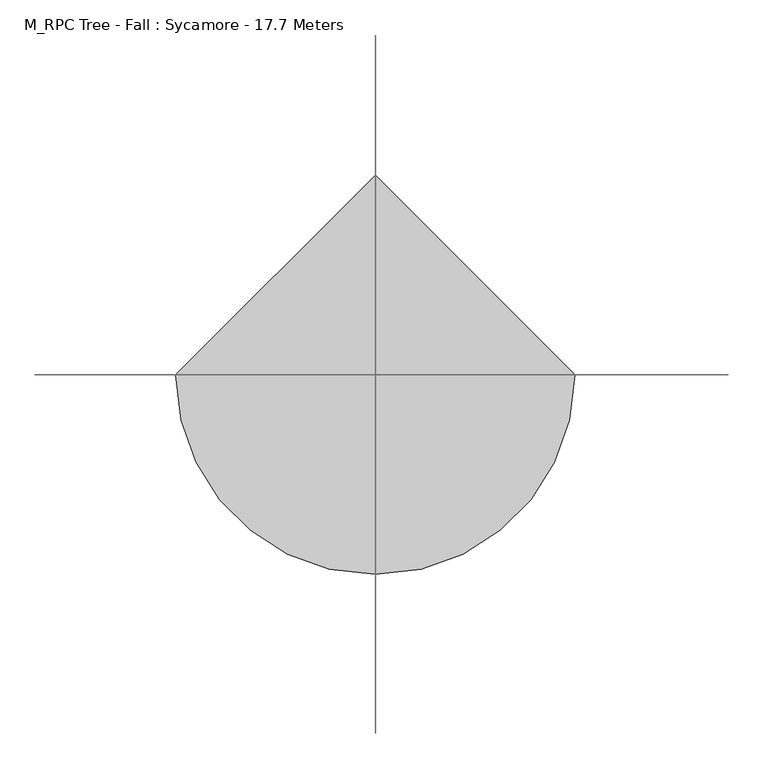
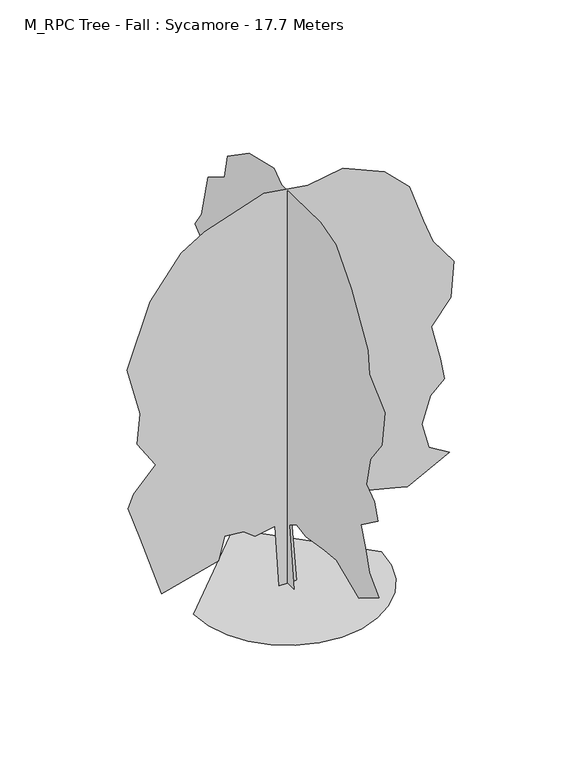
"""IFC4 building model written with IfcOpenShell, lengths in millimetres: geographic element geometry, M_RPC Tree - Fall : Sycamore - 17.7 Meters."""

from ifc_helpers import new_model, si_unit, origin, place, context, project, spatial, triangles, source, transform, mapped, element, save


def m_rpc_tree_fall_sycamore_17_7_meters_35b6092d(model_context):
    return source(origin(), model_context, "Body", "Tessellation", [
        triangles([(-349.2535366, 1.53e-05, 0.0), (-516.9583074, -0.0002974, 2684.3285934), (-1359.4699265, -0.0002437, 2543.0828545), (-1839.0104233, -0.0002655, 2901.4063316), (-2629.9138916, -0.0002406, 2982.7757835), (-2874.1989807, -0.0001124, 1997.0510674), (-5250.1434906, 6.53e-05, 1377.9031036), (-6147.3555862, -0.000224, 4133.6032127), (-6660.0481293, -0.0003773, 5607.5821381), (-6417.9123276, -0.0004558, 6177.2432968), (-5506.4894714, -0.0006111, 7145.6597672), (-6275.5285767, -0.0007188, 8331.2298431), (-6147.3555862, -0.0008772, 9612.9614914), (-6692.0851273, -0.0011055, 11727.8062408), (-5730.7990356, -0.0014684, 14419.4163666), (-4433.1375458, -0.0017257, 16101.5729919), (-3455.7445885, -0.0018391, 16694.4716858), (-988.4251328, -0.0020462, 17527.584787), (851.3210741, -0.0020939, 17252.7794678), (2312.012075, -0.0021854, 17484.8769287), (4042.347155, -0.0021706, 16726.5081024), (5099.7439499, -0.0020946, 15701.1485962), (5676.5360687, -0.0019174, 14002.8603973), (6061.0556213, -0.0018081, 12945.4377319), (6935.6115417, -0.0017068, 11774.5336212), (6830.0691467, -0.0015171, 10221.7900269), (5996.9560455, -0.0013584, 9196.4049408), (6384.9143417, -0.0011933, 7668.9220139), (6541.6855865, -0.0010881, 6729.0782181), (5964.9190475, -0.0009979, 6184.3486771), (5612.4364929, -0.000845, 5030.8155991), (5910.7322388, -0.0007264, 3926.7664192), (6763.6435501, -0.0007002, 3394.2497955), (5003.6329559, -0.0005166, 2499.4093575), (4490.9407036, -0.0005095, 2627.5875801), (2696.5165123, -0.0004845, 3076.1811287), (1440.3840282, -0.0004033, 2855.1082855), (1094.3746977, -0.0003954, 2915.9708496), (154.1243679, -0.0004206, 3471.9020325), (137.1452807, -0.000361, 2978.527787), (372.6680594, -1.63e-05, 0.0005185), (-4.17e-05, -471.0243379, 0.2782564), (8.77e-05, -141.3566061, 2629.9391808), (4.63e-05, -652.0445749, 2979.1850143), (-2.35e-05, -1323.5161617, 2841.0242615), (-0.0001758, -2683.2667397, 3076.4593094), (-0.0002438, -3532.3602608, 3156.5390144), (-0.0004492, -5182.6051712, 2467.6429825), (-0.0005761, -6624.5468079, 3364.8425789), (-0.0004815, -5919.6072784, 4037.7451103), (-0.0004283, -5631.2242996, 4966.9944946), (-0.0003779, -5310.778743, 5800.1070145), (-0.0004606, -6528.4363953, 6697.3191101), (-0.00042, -6304.1268311, 7402.2592209), (-0.0003408, -5695.2977142, 7818.84077), (-0.0003318, -5983.6812744, 9100.5468384), (-0.0003879, -6816.8193741, 10222.0679169), (-0.0003635, -7041.1033585, 11792.1581268), (-0.0002023, -5935.4865417, 12801.0825897), (-0.0001876, -5823.471286, 13810.8663025), (1.84e-05, -4637.8756302, 15765.5004822), (0.0001578, -3516.3795502, 17047.2315491), (0.0002895, -2398.0845829, 17367.6526886), (0.000582, 424.9133443, 17303.5786926), (0.0006581, 985.041909, 17699.9824036), (0.0008215, 2791.8435425, 17271.5166962), (0.0009453, 4321.0714211, 16214.0940308), (0.0009433, 4550.9940147, 15152.9541504), (0.0010322, 5744.0488083, 14419.6954193), (0.0010379, 6224.7043533, 12497.1232361), (0.0010611, 6673.2979019, 11792.1581268), (0.0009838, 6141.0594589, 11343.5645782), (0.0009196, 6128.5683609, 9100.5468384), (0.0009162, 6192.6673553, 8171.2977448), (0.000802, 5423.6282501, 7113.8756607), (0.0008749, 6481.0509155, 6152.5895691), (0.0008939, 6673.2979019, 5607.8600281), (0.0007251, 6000.3953705, 3204.6322998), (0.0006567, 5326.1266434, 2314.267606), (0.0006153, 5241.0911362, 1451.9952381), (0.000451, 3468.9940704, 1826.7822453), (0.0003683, 2828.1538261, 2147.2126865), (0.0003977, 2635.8812599, 3012.3853134), (0.0002491, 1386.2069572, 2435.6010429), (0.0002116, 1103.6115612, 2647.942733), (0.0001461, 454.7074923, 2583.9951828), (6.49e-05, 394.1356081, 0.27836), (-3922.0632179, -8e-07, 0.2416303), (-3818.3919296, -898.6786486, 0.2415188), (-3523.080304, -1723.9706429, 0.2414075), (-3059.8210808, -2452.2314232, 0.2413003), (-2452.2314232, -3059.8210808, 0.2412014), (-1723.9706429, -3523.080304, 0.2411142), (-898.6786486, -3818.3919296, 0.2410432), (0.0001856, -3922.0632179, 0.2409913), (898.6786486, -3818.3919296, 0.2415145), (1723.9706429, -3523.080304, 0.2415137), (2452.2314232, -3059.8210808, 0.241537), (3059.8210808, -2452.2314232, 0.241583), (3523.080304, -1723.9706429, 0.2416495), (3818.3919296, -898.6786486, 0.241735), (3922.0632179, 0.0003428, 0.2412874), (-0.0005028, 3922.0632179, 0.2413764)], [[32, 33, 34], [41, 1, 2], [40, 41, 2], [6, 7, 8], [5, 6, 8], [32, 34, 35], [39, 40, 2], [31, 32, 35], [31, 35, 36], [28, 29, 30], [5, 8, 9], [5, 9, 10], [5, 10, 11], [4, 5, 11], [2, 3, 4], [39, 2, 4], [39, 4, 11], [24, 25, 26], [24, 26, 27], [30, 31, 36], [11, 12, 13], [39, 11, 13], [13, 14, 15], [39, 13, 15], [39, 15, 16], [39, 16, 17], [39, 17, 18], [39, 18, 19], [39, 19, 20], [39, 20, 21], [39, 21, 22], [39, 22, 23], [39, 23, 24], [39, 24, 27], [39, 27, 28], [39, 28, 30], [39, 30, 36], [39, 36, 37], [38, 39, 37], [48, 49, 50], [79, 80, 81], [86, 87, 42], [86, 42, 43], [47, 48, 50], [47, 50, 51], [70, 71, 72], [52, 53, 54], [52, 54, 55], [47, 51, 52], [83, 84, 85], [57, 58, 59], [56, 57, 59], [81, 82, 83], [79, 81, 83], [78, 79, 83], [77, 78, 83], [76, 77, 83], [75, 76, 83], [46, 47, 52], [64, 65, 66], [68, 69, 70], [66, 67, 68], [64, 66, 68], [75, 83, 85], [75, 85, 86], [75, 86, 43], [75, 43, 44], [73, 74, 75], [68, 70, 72], [64, 68, 72], [63, 64, 72], [63, 72, 73], [63, 73, 75], [63, 75, 44], [62, 63, 44], [61, 62, 44], [60, 61, 44], [59, 60, 44], [56, 59, 44], [55, 56, 44], [52, 55, 44], [46, 52, 44], [45, 46, 44], [102, 103, 88], [101, 102, 88], [101, 88, 89], [100, 101, 89], [100, 89, 90], [100, 90, 91], [99, 100, 91], [98, 99, 91], [98, 91, 92], [98, 92, 93], [98, 93, 94], [98, 94, 95], [98, 95, 96], [98, 96, 97]], closed=False),
    ])


if __name__ == "__main__":
    model = new_model("IFC4")
    model_context = context("Model", 3, world=origin())
    ifc_project = project(units=[si_unit("LENGTHUNIT", "METRE", prefix="MILLI")], contexts=[model_context])
    site = spatial("IfcSite", under=ifc_project)
    building = spatial("IfcBuilding", under=site)
    placement = place(None, origin())
    m_rpc_tree_fall_sycamore_17_7_meters_shape = m_rpc_tree_fall_sycamore_17_7_meters_35b6092d(model_context)
    element("IfcGeographicElement", 1, ObjectType="M_RPC Tree - Fall : Sycamore - 17.7 Meters", at=placement, inside=building, context=model_context, shape_type="MappedRepresentation", body=[
        mapped(m_rpc_tree_fall_sycamore_17_7_meters_shape, transform((0.0, 0.0, 0.0), x_axis=(1.0, 0.0, 0.0), y_axis=(0.0, 1.0, 0.0), z_axis=(0.0, 0.0, 1.0))),
    ])
    save(model, "model.ifc")

# Revit data of these elements
# Type "M_RPC Tree - Fall : Sycamore - 17.7 Meters"
#   built-in parameter 1005198 = "{2, 15},{39, RPC-16-G0VS-NDQ0-MUDG-8000-ST1L-LVER-AU},{1, 0},{1, 0},{2, 13},{1, 8},{5, Color},{1, 0},{1, 0},{3, 0.8},{3, 0.8},{3, 0.8},{1, 8},{7, BBoxMin},{1, 0},{1, 0},{1, 0},{1, 0},{1, 0},{1, 8},{7, BBoxMax},{1, 0},{1, 0},{1, 0},{1, 0},{1, 0},{2, 11},{9, RPCTypeId},{1, 0},{1, 0},{39, RPC-16-G0VS-NDQ0-MUDG-8000-ST1L-LVER-AU},{1, 6},{14, RPCPlantHeight},{1, 0},{1, 0},{7, 58.0709},{2, 11},{7, keyword},{1, 0},{1, 0},{39, :RPCs:Fall Trees [General]:Geometry:RPC},{2, 11},{8, category},{1, 0},{1, 0},{20, Fall Trees [General]},{2, 11},{12, LocalizedUID},{1, 0},{1, 0},{15, Sycamore [Fall]},{2, 14},{6, Height},{1, 0},{1, 0},{7, 58.0709},{1, 2},{16, Cast Reflections},{1, 0},{1, 0},{1, 0},{1, 2},{12, Cast Shadows},{1, 0},{1, 0},{1, 1},{1, 2},{9, Lock View},{1, 0},{1, 0},{1, 0},{1, 4},{5, ViewC},{1, 0},{1, 0},{1, 0},{21, assetlibrary_base.fbx},{1, 5},"
#   built-in parameter 1005195 = "RPC-16-G0VS-NDQ0-MUDG-8000-ST1L-LVER-AU"
#   Type Comments = "Sycamore"
#   Height = 17.7 m
#   Default Elevation = 0
